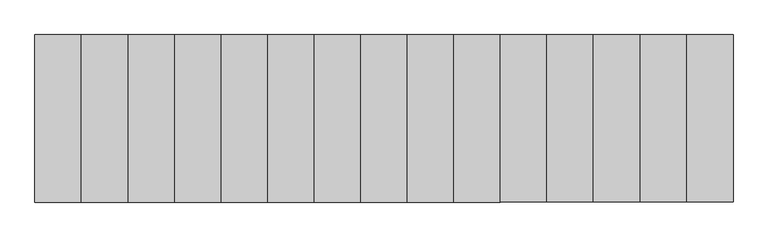
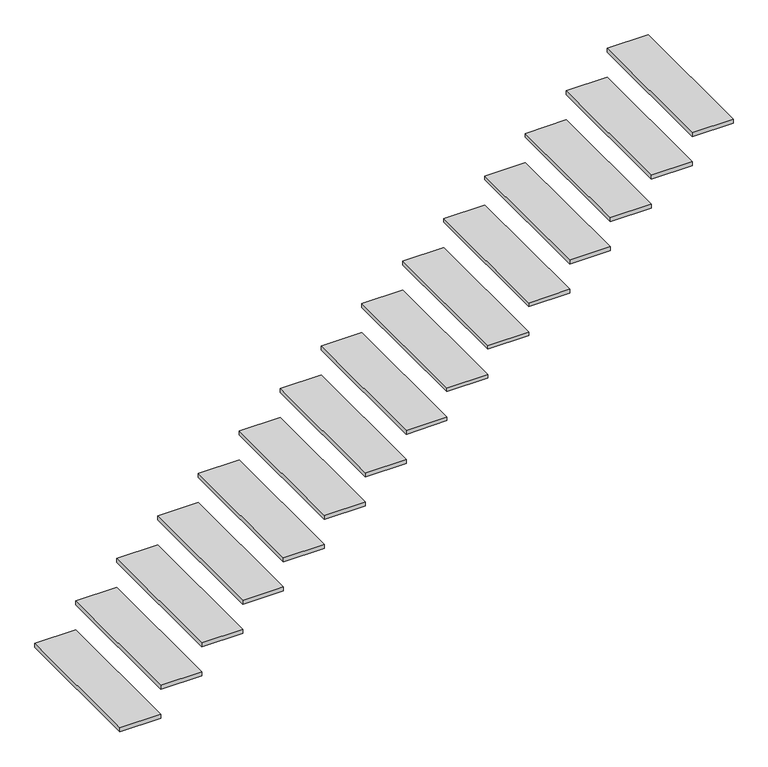
"""IFC4 building model written with IfcOpenShell, lengths in millimetres: stair flight geometry."""

import ifcopenshell
import ifcopenshell.guid

model = None  # the IFC model being written
_history = None  # IfcOwnerHistory: only IFC2X3 demands one
_inside = {}  # id of a spatial element -> (the spatial element, [elements in it])
_under = {}  # id of a project, library or spatial element -> (it, [spatial elements below it])
_declared = {}  # id of a project -> (the project, [libraries it declares])
_typed = {}  # id of a type object -> (the type object, [elements of that type])
_made_of = {}  # id of a material, layer set ... -> (it, [elements and type objects made of it])


def new_model(schema):
    """Start an empty IFC model of exactly this schema.

    Asked for "IFC4X3", IfcOpenShell would pick the latest addendum, in which some entities
    have other attributes; the version numbers below select the first issue.
    IFC2X3 requires an IfcOwnerHistory on every rooted entity: one is made here for all.
    """
    global model, _history
    if schema == "IFC4X3":
        model = ifcopenshell.file(schema_version=(4, 3, 0, 0))
    else:
        model = ifcopenshell.file(schema=schema)
    _inside.clear()
    _under.clear()
    _declared.clear()
    _typed.clear()
    _made_of.clear()
    _history = None
    if model.schema == "IFC2X3":
        org = make("IfcOrganization", Name="unknown")
        user = make(
            "IfcPersonAndOrganization",
            ThePerson=make("IfcPerson", FamilyName="unknown"),
            TheOrganization=org,
        )
        app = make(
            "IfcApplication",
            ApplicationDeveloper=org,
            Version="unknown",
            ApplicationFullName="unknown",
            ApplicationIdentifier="unknown",
        )
        _history = make(
            "IfcOwnerHistory",
            OwningUser=user,
            OwningApplication=app,
            ChangeAction="ADDED",
            CreationDate=0,
        )
    return model


def make(cls, **values):
    """One entity of the class cls with the attributes given. An attribute that is None is left unset."""
    return model.create_entity(
        cls, **{name: value for name, value in values.items() if value is not None}
    )


def rooted(cls, **values):
    """An entity with a GlobalId (a new one), such as an element, a storey or a relation."""
    return make(cls, GlobalId=ifcopenshell.guid.new(), OwnerHistory=_history, **values)


def si_unit(unit_type, name, prefix=None):
    """IfcSIUnit, for example si_unit("LENGTHUNIT", "METRE", prefix="MILLI")."""
    return make("IfcSIUnit", UnitType=unit_type, Prefix=prefix, Name=name)


def assignment(units):
    """IfcUnitAssignment: the units of a project."""
    return None if units is None else make("IfcUnitAssignment", Units=units)


def point(xyz):
    """IfcCartesianPoint."""
    return None if xyz is None else make("IfcCartesianPoint", Coordinates=xyz)


def direction(xyz):
    """IfcDirection."""
    return None if xyz is None else make("IfcDirection", DirectionRatios=xyz)


def frame(location, z_axis=None, x_axis=None):
    """IfcAxis2Placement3D, a coordinate frame: its origin and axes. An axis left out is left unset."""
    return make(
        "IfcAxis2Placement3D",
        Location=point(location),
        Axis=direction(z_axis),
        RefDirection=direction(x_axis),
    )


def origin():
    """The frame at (0, 0, 0) with its axes left unset."""
    return frame((0.0, 0.0, 0.0))


def place(relative_to, where):
    """IfcLocalPlacement: puts the frame where relative to a parent placement (None: the world)."""
    return make(
        "IfcLocalPlacement", PlacementRelTo=relative_to, RelativePlacement=where
    )


def context(
    kind, dimensions, precision=None, world=None, true_north=None, identifier=None
):
    """IfcGeometricRepresentationContext, for example the 3D "Model" context."""
    return make(
        "IfcGeometricRepresentationContext",
        ContextIdentifier=identifier,
        ContextType=kind,
        CoordinateSpaceDimension=dimensions,
        Precision=precision,
        WorldCoordinateSystem=world,
        TrueNorth=true_north,
    )


def project(units=None, contexts=None):
    """IfcProject with its units and contexts."""
    return rooted(
        "IfcProject",
        Name="project",
        RepresentationContexts=contexts,
        UnitsInContext=assignment(units),
    )


def spatial(cls, under=None, at=None, **own):
    """A site, building, storey or space (cls), placed at a placement, below another one or the project."""
    s = rooted(cls, ObjectPlacement=at, **own)
    if under is not None:
        _under.setdefault(under.id(), (under, []))[1].append(s)
    return s


def polyline(points):
    """IfcPolyline through the points."""
    return make("IfcPolyline", Points=[point(p) for p in points])


def outline(outer, holes=None, kind="AREA"):
    """IfcArbitraryClosedProfileDef: a profile drawn as a closed curve; with holes, ...WithVoids."""
    if holes is None:
        return make("IfcArbitraryClosedProfileDef", ProfileType=kind, OuterCurve=outer)
    return make(
        "IfcArbitraryProfileDefWithVoids",
        ProfileType=kind,
        OuterCurve=outer,
        InnerCurves=holes,
    )


def extrude(swept, where, along, depth):
    """IfcExtrudedAreaSolid: the profile swept, set in the frame where, extruded along a direction by depth."""
    return make(
        "IfcExtrudedAreaSolid",
        SweptArea=swept,
        Position=where,
        ExtrudedDirection=direction(along),
        Depth=depth,
    )


def shape(context_of_items, identifier, shape_type, items):
    """IfcShapeRepresentation: the items that make up one representation, for example the "Body"."""
    return make(
        "IfcShapeRepresentation",
        ContextOfItems=context_of_items,
        RepresentationIdentifier=identifier,
        RepresentationType=shape_type,
        Items=items,
    )


def source(mapping_origin, context_of_items, identifier, shape_type, items):
    """IfcRepresentationMap: a shape defined once, which mapped items show again and again."""
    return make(
        "IfcRepresentationMap",
        MappingOrigin=mapping_origin,
        MappedRepresentation=shape(context_of_items, identifier, shape_type, items),
    )


def transform(
    local_origin,
    x_axis=None,
    y_axis=None,
    z_axis=None,
    scale=None,
    scale2=None,
    scale3=None,
    uniform=True,
):
    """IfcCartesianTransformationOperator3D, or its non-uniform kind. x_axis, y_axis, z_axis: its Axis1, 2, 3."""
    if uniform:
        return make(
            "IfcCartesianTransformationOperator3D",
            Axis1=direction(x_axis),
            Axis2=direction(y_axis),
            LocalOrigin=point(local_origin),
            Scale=scale,
            Axis3=direction(z_axis),
        )
    return make(
        "IfcCartesianTransformationOperator3DnonUniform",
        Axis1=direction(x_axis),
        Axis2=direction(y_axis),
        LocalOrigin=point(local_origin),
        Scale=scale,
        Axis3=direction(z_axis),
        Scale2=scale2,
        Scale3=scale3,
    )


def mapped(mapping_source, mapping_target):
    """IfcMappedItem: shows the shape of a source again, moved by a transform."""
    return make(
        "IfcMappedItem", MappingSource=mapping_source, MappingTarget=mapping_target
    )


def made_of(thing, what):
    """Note that an element or type object is made of a material, layer set ...; save() writes the relation."""
    if what is not None:
        _made_of.setdefault(what.id(), (what, []))[1].append(thing)
    return thing


def element(
    cls,
    number,
    at=None,
    inside=None,
    cuts=None,
    type_object=None,
    material=None,
    context=None,
    identifier="Body",
    shape_type=None,
    held_by="IfcProductDefinitionShape",
    body=None,
    shapes=None,
    **own,
):
    """One element of the class cls, such as IfcWall. Its Tag is "e" and its number.

    at: its placement. inside: the storey or other place that contains it. cuts: it is an
    opening in that element (IfcRelVoidsElement). A single representation is given by context,
    identifier, shape_type and body (its items); several are given by shapes. held_by: the class
    of the entity that holds the representations. save() writes the other relations.
    """
    e = rooted(cls, Tag="e%d" % number, ObjectPlacement=at, **own)
    if body is not None:
        shapes = [shape(context, identifier, shape_type, body)]
    if shapes is not None:
        e.Representation = make(held_by, Representations=shapes)
    if inside is not None:
        _inside.setdefault(inside.id(), (inside, []))[1].append(e)
    if cuts is not None:
        rooted(
            "IfcRelVoidsElement", RelatingBuildingElement=cuts, RelatedOpeningElement=e
        )
    if type_object is not None:
        _typed.setdefault(type_object.id(), (type_object, []))[1].append(e)
    return made_of(e, material)


def aggregate(whole, parts):
    """IfcRelAggregates: a whole, such as a stair, and the parts it consists of."""
    return rooted("IfcRelAggregates", RelatingObject=whole, RelatedObjects=parts)


def save(model, path):
    """Write the relations noted so far, then the file.

    IfcRelAggregates (storeys below a building ...), IfcRelContainedInSpatialStructure (elements
    in a storey), IfcRelDefinesByType, IfcRelAssociatesMaterial and IfcRelDeclares: one each for
    every whole, place, type object, material and project.
    """
    for whole, parts in _under.values():
        aggregate(whole, parts)
    for where, things in _inside.values():
        rooted(
            "IfcRelContainedInSpatialStructure",
            RelatedElements=things,
            RelatingStructure=where,
        )
    for kind, things in _typed.values():
        rooted("IfcRelDefinesByType", RelatedObjects=things, RelatingType=kind)
    for what, things in _made_of.values():
        rooted("IfcRelAssociatesMaterial", RelatedObjects=things, RelatingMaterial=what)
    for by, libraries in _declared.values():
        rooted("IfcRelDeclares", RelatingContext=by, RelatedDefinitions=libraries)
    model.write(path)


def stair_flight_c3952520(model_context):
    return source(origin(), model_context, "Body", "SweptSolid", [
        extrude(outline(polyline([(-26976.8481446, -16465.6871906), (-26976.8481446, -17380.0871906), (-27230.8481446, -17380.0871906), (-27230.8481446, -16465.6871906), (-26976.8481446, -16465.6871906)])), frame((0.0, 0.0, 165.1), z_axis=(0.0, 0.0, 1.0), x_axis=(1.0, 0.0, 0.0)), (0.0, 0.0, 1.0), 25.4),
        extrude(outline(polyline([(-26722.8481446, -16465.6871906), (-26722.8481446, -17380.0871906), (-26976.8481446, -17380.0871906), (-26976.8481446, -16465.6871906), (-26722.8481446, -16465.6871906)])), frame((0.0, 0.0, 355.6), z_axis=(0.0, 0.0, 1.0), x_axis=(1.0, 0.0, 0.0)), (0.0, 0.0, 1.0), 25.4),
        extrude(outline(polyline([(-26468.8481446, -16465.6871906), (-26468.8481446, -17380.0871906), (-26722.8481446, -17380.0871906), (-26722.8481446, -16465.6871906), (-26468.8481446, -16465.6871906)])), frame((0.0, 0.0, 546.1), z_axis=(0.0, 0.0, 1.0), x_axis=(1.0, 0.0, 0.0)), (0.0, 0.0, 1.0), 25.4),
        extrude(outline(polyline([(-26214.8481446, -16465.6871906), (-26214.8481446, -17380.0871906), (-26468.8481446, -17380.0871906), (-26468.8481446, -16465.6871906), (-26214.8481446, -16465.6871906)])), frame((0.0, 0.0, 736.6), z_axis=(0.0, 0.0, 1.0), x_axis=(1.0, 0.0, 0.0)), (0.0, 0.0, 1.0), 25.4),
        extrude(outline(polyline([(-25960.8481446, -16465.6871906), (-25960.8481446, -17380.0871906), (-26214.8481446, -17380.0871906), (-26214.8481446, -16465.6871906), (-25960.8481446, -16465.6871906)])), frame((0.0, 0.0, 927.1), z_axis=(0.0, 0.0, 1.0), x_axis=(1.0, 0.0, 0.0)), (0.0, 0.0, 1.0), 25.4),
        extrude(outline(polyline([(-25706.8481446, -16465.6871906), (-25706.8481446, -17380.0871906), (-25960.8481446, -17380.0871906), (-25960.8481446, -16465.6871906), (-25706.8481446, -16465.6871906)])), frame((0.0, 0.0, 1117.6), z_axis=(0.0, 0.0, 1.0), x_axis=(1.0, 0.0, 0.0)), (0.0, 0.0, 1.0), 25.4),
        extrude(outline(polyline([(-25452.8481446, -16465.6871906), (-25452.8481446, -17380.0871906), (-25706.8481446, -17380.0871906), (-25706.8481446, -16465.6871906), (-25452.8481446, -16465.6871906)])), frame((0.0, 0.0, 1308.1), z_axis=(0.0, 0.0, 1.0), x_axis=(1.0, 0.0, 0.0)), (0.0, 0.0, 1.0), 25.4),
        extrude(outline(polyline([(-25198.8481446, -16465.6871906), (-25198.8481446, -17380.0871906), (-25452.8481446, -17380.0871906), (-25452.8481446, -16465.6871906), (-25198.8481446, -16465.6871906)])), frame((0.0, 0.0, 1498.6), z_axis=(0.0, 0.0, 1.0), x_axis=(1.0, 0.0, 0.0)), (0.0, 0.0, 1.0), 25.4),
        extrude(outline(polyline([(-24944.8481446, -16465.6871906), (-24944.8481446, -17380.0871906), (-25198.8481446, -17380.0871906), (-25198.8481446, -16465.6871906), (-24944.8481446, -16465.6871906)])), frame((0.0, 0.0, 1689.1), z_axis=(0.0, 0.0, 1.0), x_axis=(1.0, 0.0, 0.0)), (0.0, 0.0, 1.0), 25.4),
        extrude(outline(polyline([(-24690.8481446, -16465.6871906), (-24690.8481446, -17380.0871906), (-24944.8481446, -17380.0871906), (-24944.8481446, -16465.6871906), (-24690.8481446, -16465.6871906)])), frame((0.0, 0.0, 1879.6), z_axis=(0.0, 0.0, 1.0), x_axis=(1.0, 0.0, 0.0)), (0.0, 0.0, 1.0), 25.4),
        extrude(outline(polyline([(-24436.8481446, -16465.6871906), (-24436.8481446, -17380.0871906), (-24690.8481446, -17380.0871906), (-24690.8481446, -16465.6871906), (-24436.8481446, -16465.6871906)])), frame((0.0, 0.0, 2070.1), z_axis=(0.0, 0.0, 1.0), x_axis=(1.0, 0.0, 0.0)), (0.0, 0.0, 1.0), 25.4),
        extrude(outline(polyline([(-24182.8481446, -16465.6871906), (-24182.8481446, -17380.0871906), (-24436.8481446, -17380.0871906), (-24436.8481446, -16465.6871906), (-24182.8481446, -16465.6871906)])), frame((0.0, 0.0, 2260.6), z_axis=(0.0, 0.0, 1.0), x_axis=(1.0, 0.0, 0.0)), (0.0, 0.0, 1.0), 25.4),
        extrude(outline(polyline([(-23928.8481446, -16465.6871906), (-23928.8481446, -17380.0871906), (-24182.8481446, -17380.0871906), (-24182.8481446, -16465.6871906), (-23928.8481446, -16465.6871906)])), frame((0.0, 0.0, 2451.1), z_axis=(0.0, 0.0, 1.0), x_axis=(1.0, 0.0, 0.0)), (0.0, 0.0, 1.0), 25.4),
        extrude(outline(polyline([(-23674.8481446, -16465.6871906), (-23674.8481446, -17380.0871906), (-23928.8481446, -17380.0871906), (-23928.8481446, -16465.6871906), (-23674.8481446, -16465.6871906)])), frame((0.0, 0.0, 2641.6), z_axis=(0.0, 0.0, 1.0), x_axis=(1.0, 0.0, 0.0)), (0.0, 0.0, 1.0), 25.4),
        extrude(outline(polyline([(-23420.8481446, -16465.6871906), (-23420.8481446, -17380.0871906), (-23674.8481446, -17380.0871906), (-23674.8481446, -16465.6871906), (-23420.8481446, -16465.6871906)])), frame((0.0, 0.0, 2832.1), z_axis=(0.0, 0.0, 1.0), x_axis=(1.0, 0.0, 0.0)), (0.0, 0.0, 1.0), 25.4),
    ])


if __name__ == "__main__":
    model = new_model("IFC4")
    model_context = context("Model", 3, world=origin())
    ifc_project = project(units=[si_unit("LENGTHUNIT", "METRE", prefix="MILLI")], contexts=[model_context])
    site = spatial("IfcSite", under=ifc_project)
    building = spatial("IfcBuilding", under=site)
    placement = place(None, origin())
    stair_flight_shape = stair_flight_c3952520(model_context)
    element("IfcStairFlight", 1, at=placement, inside=building, context=model_context, shape_type="MappedRepresentation", body=[
        mapped(stair_flight_shape, transform((0.0, 0.0, 0.0), x_axis=(1.0, 0.0, 0.0), y_axis=(0.0, 1.0, 0.0), z_axis=(0.0, 0.0, 1.0))),
    ])
    save(model, "model.ifc")

# Revit data of these elements
# Element 1 (IfcStairFlight)
#   Materials on its faces: "Wood - Cherry"
# Materials
#   "Wood - Cherry": class "Unassigned", colour RGB 226 177 128, transparency 0
